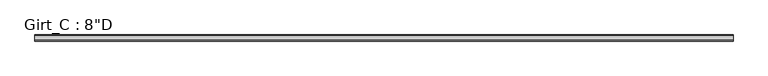
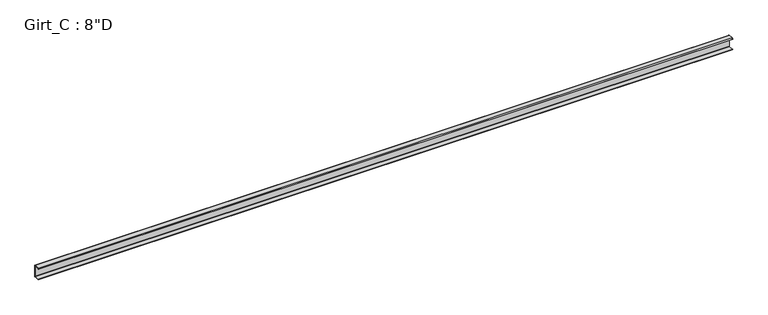
"""IFC4 building model written with IfcOpenShell, lengths in millimetres: beam geometry."""

from ifc_helpers import new_model, si_unit, point, frame, frame_2d, origin, place, context, project, spatial, polyline, circle_curve, trimmed, segment, composite_curve, outline, extrude, source, transform, mapped, element, save


def beam_ac5e974c(model_context):
    return source(origin(), model_context, "Body", "SweptSolid", [
        extrude(outline(composite_curve([segment(polyline([(-87.5109375, 101.6), (-3.3734375, 101.6)]), True, "CONTINUOUS"), segment(trimmed(circle_curve(frame_2d((-3.3734375, 96.8375)), 4.7625), [point((-3.3734375, 101.6))], [point((1.3890625, 96.8375))], False, "CARTESIAN"), True, "CONTINUOUS"), segment(polyline([(1.3890625, 96.8375), (1.3890625, -96.8375)]), True, "CONTINUOUS"), segment(trimmed(circle_curve(frame_2d((-3.3734375, -96.8375)), 4.7625), [point((1.3890625, -96.8375))], [point((-3.3734375, -101.6))], False, "CARTESIAN"), True, "CONTINUOUS"), segment(polyline([(-3.3734375, -101.6), (-87.5109375, -101.6), (-99.7792647, -86.979177), (-97.6510975, -85.1934327), (-86.2154765, -98.821875), (-3.2694106, -98.821875)]), True, "CONTINUOUS"), segment(trimmed(circle_curve(frame_2d((-3.3748024, -96.8389339)), 1.9857399), [point((-3.2694106, -98.821875))], [point((-1.3890625, -96.8389339))], True, "CARTESIAN"), True, "CONTINUOUS"), segment(polyline([(-1.3890625, -96.8389339), (-1.3890625, 96.8381931)]), True, "CONTINUOUS"), segment(trimmed(circle_curve(frame_2d((-3.3741066, 96.8381931)), 1.9850441), [point((-1.3890625, 96.8381931))], [point((-3.3005807, 98.821875))], True, "CARTESIAN"), True, "CONTINUOUS"), segment(polyline([(-3.3005807, 98.821875), (-86.2154765, 98.821875), (-97.6278742, 85.221109), (-99.7560415, 87.0068534), (-87.5109375, 101.6)]), True, "CONTINUOUS")], self_intersect=False)), frame((-5735.1929994, 0.0, 0.0), z_axis=(1.0, 0.0, 0.0), x_axis=(0.0, 1.0, 0.0)), (0.0, 0.0, 1.0), 11489.6955156),
    ])


if __name__ == "__main__":
    model = new_model("IFC4")
    model_context = context("Model", 3, world=origin())
    ifc_project = project(units=[si_unit("LENGTHUNIT", "METRE", prefix="MILLI")], contexts=[model_context])
    site = spatial("IfcSite", under=ifc_project)
    building = spatial("IfcBuilding", under=site)
    placement = place(None, origin())
    beam_shape = beam_ac5e974c(model_context)
    element("IfcBeam", 1, ObjectType="Girt_C : 8\"D", at=placement, inside=building, context=model_context, shape_type="MappedRepresentation", body=[
        mapped(beam_shape, transform((0.0, 0.0, 0.0), x_axis=(1.0, 0.0, 0.0), y_axis=(0.0, 1.0, 0.0), z_axis=(0.0, 0.0, 1.0))),
    ])
    save(model, "model.ifc")

# Revit data of these elements
# Type "Girt_C : 8\"D"
#   half leg = 0' - 1 3/4"
#   Web_Thickness = 0' - 0 7/64"
#   Length [instance default] = 10' - 0"
#   Leg_1 = 0' - 3 1/2"
#   Height = 0' - 8"
#   Structural Material [instance default] = none
# Element 1 (IfcBeam, "Girt_C : 8\"D")
#   Structural Material = GALVANIZED 'CEE' SECTION (8.0x3.5C - SEE STRUCT. DWGS)
#   Materials on its faces: "GALVANIZED 'CEE' SECTION (8.0x3.5C - SEE STRUCT. DWGS)"
# Materials
#   "GALVANIZED 'CEE' SECTION (8.0x3.5C - SEE STRUCT. DWGS)": class "Metal", colour RGB 137 146 153, transparency 0, Description = "Steel, mill finish", Cost = 0
